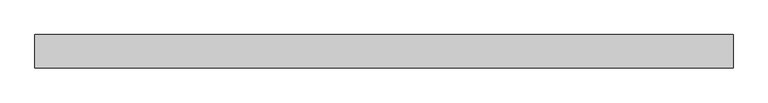
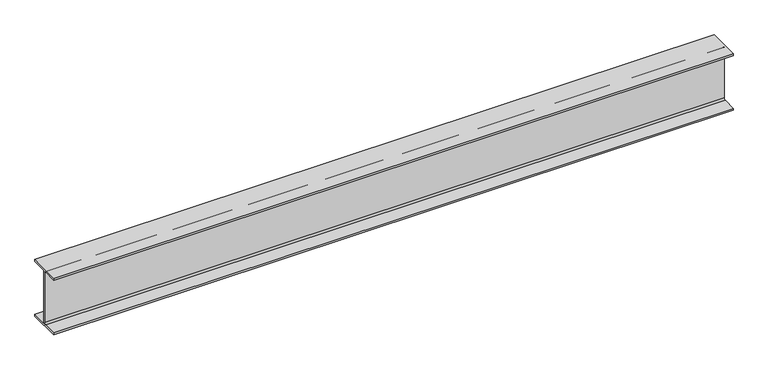
"""IFC4 building model written with IfcOpenShell, lengths in millimetres: beam geometry, Old_Steel Beam_H-KSD3502 : H_SB_ASB_H-200×200x8x12."""

import ifcopenshell
import ifcopenshell.guid

model = None  # the IFC model being written
_history = None  # IfcOwnerHistory: only IFC2X3 demands one
_inside = {}  # id of a spatial element -> (the spatial element, [elements in it])
_under = {}  # id of a project, library or spatial element -> (it, [spatial elements below it])
_declared = {}  # id of a project -> (the project, [libraries it declares])
_typed = {}  # id of a type object -> (the type object, [elements of that type])
_made_of = {}  # id of a material, layer set ... -> (it, [elements and type objects made of it])


def new_model(schema):
    """Start an empty IFC model of exactly this schema.

    Asked for "IFC4X3", IfcOpenShell would pick the latest addendum, in which some entities
    have other attributes; the version numbers below select the first issue.
    IFC2X3 requires an IfcOwnerHistory on every rooted entity: one is made here for all.
    """
    global model, _history
    if schema == "IFC4X3":
        model = ifcopenshell.file(schema_version=(4, 3, 0, 0))
    else:
        model = ifcopenshell.file(schema=schema)
    _inside.clear()
    _under.clear()
    _declared.clear()
    _typed.clear()
    _made_of.clear()
    _history = None
    if model.schema == "IFC2X3":
        org = make("IfcOrganization", Name="unknown")
        user = make(
            "IfcPersonAndOrganization",
            ThePerson=make("IfcPerson", FamilyName="unknown"),
            TheOrganization=org,
        )
        app = make(
            "IfcApplication",
            ApplicationDeveloper=org,
            Version="unknown",
            ApplicationFullName="unknown",
            ApplicationIdentifier="unknown",
        )
        _history = make(
            "IfcOwnerHistory",
            OwningUser=user,
            OwningApplication=app,
            ChangeAction="ADDED",
            CreationDate=0,
        )
    return model


def make(cls, **values):
    """One entity of the class cls with the attributes given. An attribute that is None is left unset."""
    return model.create_entity(
        cls, **{name: value for name, value in values.items() if value is not None}
    )


def rooted(cls, **values):
    """An entity with a GlobalId (a new one), such as an element, a storey or a relation."""
    return make(cls, GlobalId=ifcopenshell.guid.new(), OwnerHistory=_history, **values)


def si_unit(unit_type, name, prefix=None):
    """IfcSIUnit, for example si_unit("LENGTHUNIT", "METRE", prefix="MILLI")."""
    return make("IfcSIUnit", UnitType=unit_type, Prefix=prefix, Name=name)


def assignment(units):
    """IfcUnitAssignment: the units of a project."""
    return None if units is None else make("IfcUnitAssignment", Units=units)


def point(xyz):
    """IfcCartesianPoint."""
    return None if xyz is None else make("IfcCartesianPoint", Coordinates=xyz)


def direction(xyz):
    """IfcDirection."""
    return None if xyz is None else make("IfcDirection", DirectionRatios=xyz)


def frame(location, z_axis=None, x_axis=None):
    """IfcAxis2Placement3D, a coordinate frame: its origin and axes. An axis left out is left unset."""
    return make(
        "IfcAxis2Placement3D",
        Location=point(location),
        Axis=direction(z_axis),
        RefDirection=direction(x_axis),
    )


def frame_2d(location, x_axis=None):
    """IfcAxis2Placement2D, a coordinate frame in the plane: its origin and x axis."""
    return make(
        "IfcAxis2Placement2D", Location=point(location), RefDirection=direction(x_axis)
    )


def origin():
    """The frame at (0, 0, 0) with its axes left unset."""
    return frame((0.0, 0.0, 0.0))


def place(relative_to, where):
    """IfcLocalPlacement: puts the frame where relative to a parent placement (None: the world)."""
    return make(
        "IfcLocalPlacement", PlacementRelTo=relative_to, RelativePlacement=where
    )


def context(
    kind, dimensions, precision=None, world=None, true_north=None, identifier=None
):
    """IfcGeometricRepresentationContext, for example the 3D "Model" context."""
    return make(
        "IfcGeometricRepresentationContext",
        ContextIdentifier=identifier,
        ContextType=kind,
        CoordinateSpaceDimension=dimensions,
        Precision=precision,
        WorldCoordinateSystem=world,
        TrueNorth=true_north,
    )


def project(units=None, contexts=None):
    """IfcProject with its units and contexts."""
    return rooted(
        "IfcProject",
        Name="project",
        RepresentationContexts=contexts,
        UnitsInContext=assignment(units),
    )


def spatial(cls, under=None, at=None, **own):
    """A site, building, storey or space (cls), placed at a placement, below another one or the project."""
    s = rooted(cls, ObjectPlacement=at, **own)
    if under is not None:
        _under.setdefault(under.id(), (under, []))[1].append(s)
    return s


def polyline(points):
    """IfcPolyline through the points."""
    return make("IfcPolyline", Points=[point(p) for p in points])


def circle_curve(where, radius):
    """IfcCircle in the frame where."""
    return make("IfcCircle", Position=where, Radius=radius)


def trimmed(basis, trim1, trim2, sense, master):
    """IfcTrimmedCurve: the piece of a basis curve between two trims."""
    return make(
        "IfcTrimmedCurve",
        BasisCurve=basis,
        Trim1=trim1,
        Trim2=trim2,
        SenseAgreement=sense,
        MasterRepresentation=master,
    )


def segment(curve, same_sense, transition):
    """IfcCompositeCurveSegment."""
    return make(
        "IfcCompositeCurveSegment",
        Transition=transition,
        SameSense=same_sense,
        ParentCurve=curve,
    )


def composite_curve(segments, self_intersect=None):
    """IfcCompositeCurve: segments joined end to end."""
    return make("IfcCompositeCurve", Segments=segments, SelfIntersect=self_intersect)


def outline(outer, holes=None, kind="AREA"):
    """IfcArbitraryClosedProfileDef: a profile drawn as a closed curve; with holes, ...WithVoids."""
    if holes is None:
        return make("IfcArbitraryClosedProfileDef", ProfileType=kind, OuterCurve=outer)
    return make(
        "IfcArbitraryProfileDefWithVoids",
        ProfileType=kind,
        OuterCurve=outer,
        InnerCurves=holes,
    )


def extrude(swept, where, along, depth):
    """IfcExtrudedAreaSolid: the profile swept, set in the frame where, extruded along a direction by depth."""
    return make(
        "IfcExtrudedAreaSolid",
        SweptArea=swept,
        Position=where,
        ExtrudedDirection=direction(along),
        Depth=depth,
    )


def shape(context_of_items, identifier, shape_type, items):
    """IfcShapeRepresentation: the items that make up one representation, for example the "Body"."""
    return make(
        "IfcShapeRepresentation",
        ContextOfItems=context_of_items,
        RepresentationIdentifier=identifier,
        RepresentationType=shape_type,
        Items=items,
    )


def source(mapping_origin, context_of_items, identifier, shape_type, items):
    """IfcRepresentationMap: a shape defined once, which mapped items show again and again."""
    return make(
        "IfcRepresentationMap",
        MappingOrigin=mapping_origin,
        MappedRepresentation=shape(context_of_items, identifier, shape_type, items),
    )


def transform(
    local_origin,
    x_axis=None,
    y_axis=None,
    z_axis=None,
    scale=None,
    scale2=None,
    scale3=None,
    uniform=True,
):
    """IfcCartesianTransformationOperator3D, or its non-uniform kind. x_axis, y_axis, z_axis: its Axis1, 2, 3."""
    if uniform:
        return make(
            "IfcCartesianTransformationOperator3D",
            Axis1=direction(x_axis),
            Axis2=direction(y_axis),
            LocalOrigin=point(local_origin),
            Scale=scale,
            Axis3=direction(z_axis),
        )
    return make(
        "IfcCartesianTransformationOperator3DnonUniform",
        Axis1=direction(x_axis),
        Axis2=direction(y_axis),
        LocalOrigin=point(local_origin),
        Scale=scale,
        Axis3=direction(z_axis),
        Scale2=scale2,
        Scale3=scale3,
    )


def mapped(mapping_source, mapping_target):
    """IfcMappedItem: shows the shape of a source again, moved by a transform."""
    return make(
        "IfcMappedItem", MappingSource=mapping_source, MappingTarget=mapping_target
    )


def made_of(thing, what):
    """Note that an element or type object is made of a material, layer set ...; save() writes the relation."""
    if what is not None:
        _made_of.setdefault(what.id(), (what, []))[1].append(thing)
    return thing


def element(
    cls,
    number,
    at=None,
    inside=None,
    cuts=None,
    type_object=None,
    material=None,
    context=None,
    identifier="Body",
    shape_type=None,
    held_by="IfcProductDefinitionShape",
    body=None,
    shapes=None,
    **own,
):
    """One element of the class cls, such as IfcWall. Its Tag is "e" and its number.

    at: its placement. inside: the storey or other place that contains it. cuts: it is an
    opening in that element (IfcRelVoidsElement). A single representation is given by context,
    identifier, shape_type and body (its items); several are given by shapes. held_by: the class
    of the entity that holds the representations. save() writes the other relations.
    """
    e = rooted(cls, Tag="e%d" % number, ObjectPlacement=at, **own)
    if body is not None:
        shapes = [shape(context, identifier, shape_type, body)]
    if shapes is not None:
        e.Representation = make(held_by, Representations=shapes)
    if inside is not None:
        _inside.setdefault(inside.id(), (inside, []))[1].append(e)
    if cuts is not None:
        rooted(
            "IfcRelVoidsElement", RelatingBuildingElement=cuts, RelatedOpeningElement=e
        )
    if type_object is not None:
        _typed.setdefault(type_object.id(), (type_object, []))[1].append(e)
    return made_of(e, material)


def aggregate(whole, parts):
    """IfcRelAggregates: a whole, such as a stair, and the parts it consists of."""
    return rooted("IfcRelAggregates", RelatingObject=whole, RelatedObjects=parts)


def save(model, path):
    """Write the relations noted so far, then the file.

    IfcRelAggregates (storeys below a building ...), IfcRelContainedInSpatialStructure (elements
    in a storey), IfcRelDefinesByType, IfcRelAssociatesMaterial and IfcRelDeclares: one each for
    every whole, place, type object, material and project.
    """
    for whole, parts in _under.values():
        aggregate(whole, parts)
    for where, things in _inside.values():
        rooted(
            "IfcRelContainedInSpatialStructure",
            RelatedElements=things,
            RelatingStructure=where,
        )
    for kind, things in _typed.values():
        rooted("IfcRelDefinesByType", RelatedObjects=things, RelatingType=kind)
    for what, things in _made_of.values():
        rooted("IfcRelAssociatesMaterial", RelatedObjects=things, RelatingMaterial=what)
    for by, libraries in _declared.values():
        rooted("IfcRelDeclares", RelatingContext=by, RelatedDefinitions=libraries)
    model.write(path)


def beam_9a6c1f0b(model_context):
    return source(origin(), model_context, "Body", "SweptSolid", [
        extrude(outline(composite_curve([segment(polyline([(82.5, -141.5), (82.5, -151.7), (-82.5, -151.7), (-82.5, -141.5), (-11.9, -141.5)]), True, "CONTINUOUS"), segment(trimmed(circle_curve(frame_2d((-11.9, -132.6)), 8.9), [point((-11.9, -141.5))], [point((-3.0, -132.6))], True, "CARTESIAN"), True, "CONTINUOUS"), segment(polyline([(-3.0, -132.6), (-3.0, 132.6)]), True, "CONTINUOUS"), segment(trimmed(circle_curve(frame_2d((-11.9, 132.6)), 8.9), [point((-3.0, 132.6))], [point((-11.9, 141.5))], True, "CARTESIAN"), True, "CONTINUOUS"), segment(polyline([(-11.9, 141.5), (-82.5, 141.5), (-82.5, 151.7), (82.5, 151.7), (82.5, 141.5), (11.9, 141.5)]), True, "CONTINUOUS"), segment(trimmed(circle_curve(frame_2d((11.9, 132.6)), 8.9), [point((11.9, 141.5))], [point((3.0, 132.6))], True, "CARTESIAN"), True, "CONTINUOUS"), segment(polyline([(3.0, 132.6), (3.0, -132.6)]), True, "CONTINUOUS"), segment(trimmed(circle_curve(frame_2d((11.9, -132.6)), 8.9), [point((3.0, -132.6))], [point((11.9, -141.5))], True, "CARTESIAN"), True, "CONTINUOUS"), segment(polyline([(11.9, -141.5), (82.5, -141.5)]), True, "CONTINUOUS")], self_intersect=False)), frame((-1601.8217098, 0.0, 0.0), z_axis=(1.0, 0.0, 0.0), x_axis=(0.0, 1.0, 0.0)), (0.0, 0.0, 1.0), 3433.6669039),
    ])


if __name__ == "__main__":
    model = new_model("IFC4")
    model_context = context("Model", 3, world=origin())
    ifc_project = project(units=[si_unit("LENGTHUNIT", "METRE", prefix="MILLI")], contexts=[model_context])
    site = spatial("IfcSite", under=ifc_project)
    building = spatial("IfcBuilding", under=site)
    placement = place(None, origin())
    beam_shape = beam_9a6c1f0b(model_context)
    element("IfcBeam", 1, ObjectType="Old_Steel Beam_H-KSD3502 : H_SB_ASB_H-200×200x8x12", at=placement, inside=building, context=model_context, shape_type="MappedRepresentation", body=[
        mapped(beam_shape, transform((0.0, 0.0, 0.0), x_axis=(1.0, 0.0, 0.0), y_axis=(0.0, 1.0, 0.0), z_axis=(0.0, 0.0, 1.0))),
    ])
    save(model, "model.ifc")

# Revit data of these elements
# Type "Old_Steel Beam_H-KSD3502 : H_SB_ASB_H-200×200x8x12"
#   Width = 20.0 cm
#   Web Thickness = 0.8 cm
#   Web Fillet = 1.3 cm
#   Warping Constant = 141376.0 cm⁶
#   Torsional Moment of Inertia = 26.2485 cm⁴
#   Torsional Modulus = 1.0 cm³
#   Section Area = 63.53 cm²
#   Plastic Modulus weak axis = 244.0 cm³
#   Plastic Modulus strong axis = 525.0 cm³
#   Perimeter = 1.16 m²/m
#   Nominal Weight = 49.90 kgf/m
#   Moment of Inertia weak axis = 1600.00 cm⁴
#   Moment of Inertia strong axis = 4720.00 cm⁴
#   Height = 20.0 cm
#   Flange Thickness = 1.2 cm
#   Elastic Modulus weak axis = 160.0 cm³
#   Elastic Modulus strong axis = 472.0 cm³
#   Centroid Vertical = 10.0 cm
#   Centroid Horizontal = 10.0 cm
#   Length [instance default] = 1.5240 m
#   Structural Material [instance default] = Steel, 45-345
#   Assembly Code = ""
# Element 1 (IfcBeam, "Old_Steel Beam_H-KSD3502 : H_SB_ASB_H-200×200x8x12")
#   Structural Material = none
# Materials
#   "Steel, 45-345": class "Metal", colour RGB 189 187 185, transparency 0, Description = "Steel 345 MPa", Cost = 0
